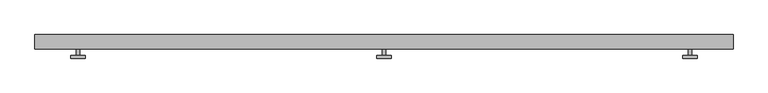
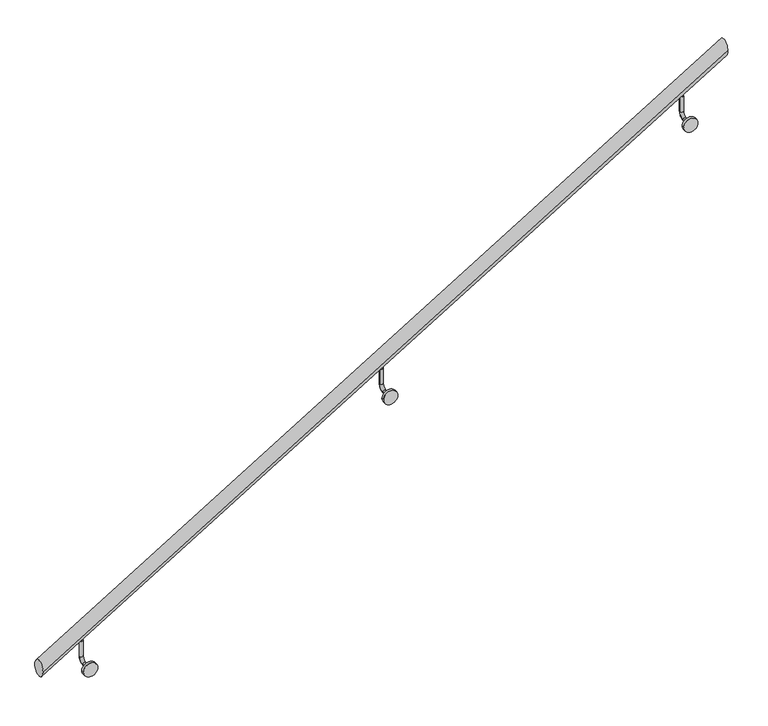
"""IFC4 building model written with IfcOpenShell, lengths in millimetres: railing geometry."""

from ifc_helpers import new_model, si_unit, point, frame, frame_2d, origin, place, context, project, spatial, circle_curve, ellipse_curve, trimmed, segment, composite_curve, outline, extrude, source, transform, mapped, element, save
from ifc_brep_helpers import plane_surface, cylinder_surface, revolved_surface, advanced_brep


def railing_4a983a7b(model_context):
    return source(origin(), model_context, "Body", "SolidModel", [
        advanced_brep(
        [(-49951.9507433, -7327.4994487, 6347.3929686), (-49951.9507433, -7377.4994487, 6347.3929686), (-47521.9507433, -7327.4994487, 7827.7377962), (-47521.9507433, -7377.4994487, 7827.7377962)],
        [
            (0, 1, ellipse_curve(frame((-49951.9507433, -7352.4994487, 6347.3929686), z_axis=(-1.0, 0.0, 0.0), x_axis=(0.0, 0.0, -1.0)), 29.2736981, 25.0)),
            (1, 0, ellipse_curve(frame((-49951.9507433, -7352.4994487, 6347.3929686), z_axis=(-1.0, 0.0, 0.0), x_axis=(0.0, 0.0, -1.0)), 29.2736981, 25.0)),
            (2, 3, ellipse_curve(frame((-47521.9507433, -7352.4994487, 7827.7377962), z_axis=(1.0, 0.0, 0.0), x_axis=(0.0, 0.0, -1.0)), 29.2736981, 25.0)),
            (3, 2, ellipse_curve(frame((-47521.9507433, -7352.4994487, 7827.7377962), z_axis=(1.0, 0.0, 0.0), x_axis=(0.0, 0.0, -1.0)), 29.2736981, 25.0)),
            (0, 2),
            (3, 1),
        ],
        [
            plane_surface(frame((-49951.9507433, -7352.4994487, 6376.6666667), z_axis=(-1.0, 0.0, 0.0), x_axis=(0.0, 1.0, 0.0))),
            plane_surface(frame((-47521.9507433, -7352.4994487, 7857.0114943), z_axis=(1.0, 0.0, 0.0), x_axis=(0.0, 1.0, 0.0))),
            cylinder_surface(frame((-49938.9442852, -7352.4994487, 6355.316443), z_axis=(-0.8540089447440427, 0.0, -0.5202583226601635), x_axis=(0.0, -1.0, 0.0)), 25.0),
        ],
        [
            (0, [[1, 2]]),
            (1, [[3, 4]]),
            (2, [[-1, 5, -4, 6]]),
            (2, [[-2, -6, -3, -5]]),
        ],
    ),
        advanced_brep(
        [(-48743.3007433, -7352.4994487, 7047.7890805), (-48730.6007433, -7352.4994487, 7047.7890805), (-48743.3007433, -7352.4994487, 6990.6390805), (-48730.6007433, -7352.4994487, 6990.6390805), (-48730.6007433, -7371.5494487, 6971.5890805), (-48743.3007433, -7371.5494487, 6971.5890805), (-48743.3007433, -7400.1244487, 6971.5890805), (-48730.6007433, -7400.1244487, 6971.5890805)],
        [
            (0, 1, circle_curve(frame((-48736.9507433, -7352.4994487, 7047.7890805), z_axis=(0.0, 0.0, 1.0), x_axis=(1.0, 0.0, 0.0)), 6.35)),
            (1, 0, circle_curve(frame((-48736.9507433, -7352.4994487, 7047.7890805), z_axis=(0.0, 0.0, 1.0), x_axis=(1.0, 0.0, 0.0)), 6.35)),
            (0, 2),
            (2, 3, circle_curve(frame((-48736.9507433, -7352.4994487, 6990.6390805), z_axis=(0.0, 0.0, 1.0), x_axis=(1.0, 0.0, 0.0)), 6.35)),
            (3, 1),
            (3, 2, circle_curve(frame((-48736.9507433, -7352.4994487, 6990.6390805), z_axis=(0.0, 0.0, 1.0), x_axis=(1.0, 0.0, 0.0)), 6.35)),
            (4, 3, circle_curve(frame((-48730.6007433, -7371.5494487, 6990.6390805), z_axis=(1.0, 0.0, 0.0), x_axis=(0.0, 1.0, 0.0)), 19.05)),
            (2, 5, circle_curve(frame((-48743.3007433, -7371.5494487, 6990.6390805), z_axis=(-1.0, 0.0, 0.0), x_axis=(0.0, 1.0, 0.0)), 19.05)),
            (5, 4, circle_curve(frame((-48736.9507433, -7371.5494487, 6971.5890805), z_axis=(0.0, 1.0, 0.0), x_axis=(1.0, 0.0, 0.0)), 6.35)),
            (4, 5, circle_curve(frame((-48736.9507433, -7371.5494487, 6971.5890805), z_axis=(0.0, 1.0, 0.0), x_axis=(1.0, 0.0, 0.0)), 6.35)),
            (6, 7, circle_curve(frame((-48736.9507433, -7400.1244487, 6971.5890805), z_axis=(0.0, -1.0, 0.0), x_axis=(1.0, 0.0, 0.0)), 6.35)),
            (7, 6, circle_curve(frame((-48736.9507433, -7400.1244487, 6971.5890805), z_axis=(0.0, -1.0, 0.0), x_axis=(1.0, 0.0, 0.0)), 6.35)),
            (5, 6),
            (7, 4),
        ],
        [
            plane_surface(frame((-48730.6007433, -7352.4994487, 7047.7890805), z_axis=(0.0, 0.0, 1.0), x_axis=(0.0, -1.0, 0.0))),
            cylinder_surface(frame((-48736.9507433, -7352.4994487, 7047.7890805), z_axis=(0.0, 0.0, 1.0), x_axis=(1.0, 0.0, 0.0)), 6.35),
            revolved_surface(trimmed(ellipse_curve(frame((-48736.9507433, -7352.4994487, 6990.6390805), z_axis=(0.0, 0.0, 1.0), x_axis=(1.0, 0.0, 0.0)), 6.35, 6.35), [point((-48743.3007433, -7352.4994487, 6990.6390805))], [point((-48730.6007433, -7352.4994487, 6990.6390805))], True, "CARTESIAN"), (-48736.9507433, -7371.5494487, 6990.6390805), (-1.0, 0.0, 0.0)),
            revolved_surface(trimmed(ellipse_curve(frame((-48736.9507433, -7352.4994487, 6990.6390805), z_axis=(0.0, 0.0, 1.0), x_axis=(1.0, 0.0, 0.0)), 6.35, 6.35), [point((-48730.6007433, -7352.4994487, 6990.6390805))], [point((-48743.3007433, -7352.4994487, 6990.6390805))], True, "CARTESIAN"), (-48736.9507433, -7371.5494487, 6990.6390805), (-1.0, 0.0, 0.0)),
            plane_surface(frame((-48736.9507433, -7400.1244487, 6965.2390805), z_axis=(0.0, -1.0, 0.0), x_axis=(1.0, 0.0, 0.0))),
            cylinder_surface(frame((-48736.9507433, -7371.5494487, 6971.5890805), z_axis=(0.0, 1.0, 0.0), x_axis=(1.0, 0.0, 0.0)), 6.35),
        ],
        [
            (0, [[1, 2]]),
            (1, [[-1, 3, 4, 5]]),
            (1, [[-2, -5, 6, -3]]),
            (2, [[7, -4, 8, 9]]),
            (3, [[-8, -6, -7, 10]]),
            (4, [[11, 12]]),
            (5, [[-9, 13, -12, 14]]),
            (5, [[-10, -14, -11, -13]]),
        ],
    ),
        extrude(outline(composite_curve([segment(trimmed(circle_curve(frame_2d((6971.5890805, -48736.9507433)), 25.4), [point((6971.5890805, -48711.5507433))], [point((6971.5890805, -48762.3507433))], False, "CARTESIAN"), True, "CONTINUOUS"), segment(trimmed(circle_curve(frame_2d((6971.5890805, -48736.9507433)), 25.4), [point((6971.5890805, -48762.3507433))], [point((6971.5890805, -48711.5507433))], False, "CARTESIAN"), True, "CONTINUOUS")], self_intersect=False)), frame((0.0, -7409.6494487, 0.0), z_axis=(0.0, 1.0, 0.0), x_axis=(0.0, 0.0, 1.0)), (0.0, 0.0, 1.0), 9.525),
        advanced_brep(
        [(-47678.3007433, -7352.4994487, 7696.5821839), (-47665.6007433, -7352.4994487, 7696.5821839), (-47678.3007433, -7352.4994487, 7639.4321839), (-47665.6007433, -7352.4994487, 7639.4321839), (-47665.6007433, -7371.5494487, 7620.3821839), (-47678.3007433, -7371.5494487, 7620.3821839), (-47678.3007433, -7400.1244487, 7620.3821839), (-47665.6007433, -7400.1244487, 7620.3821839)],
        [
            (0, 1, circle_curve(frame((-47671.9507433, -7352.4994487, 7696.5821839), z_axis=(0.0, 0.0, 1.0), x_axis=(1.0, 0.0, 0.0)), 6.35)),
            (1, 0, circle_curve(frame((-47671.9507433, -7352.4994487, 7696.5821839), z_axis=(0.0, 0.0, 1.0), x_axis=(1.0, 0.0, 0.0)), 6.35)),
            (0, 2),
            (2, 3, circle_curve(frame((-47671.9507433, -7352.4994487, 7639.4321839), z_axis=(0.0, 0.0, 1.0), x_axis=(1.0, 0.0, 0.0)), 6.35)),
            (3, 1),
            (3, 2, circle_curve(frame((-47671.9507433, -7352.4994487, 7639.4321839), z_axis=(0.0, 0.0, 1.0), x_axis=(1.0, 0.0, 0.0)), 6.35)),
            (4, 3, circle_curve(frame((-47665.6007433, -7371.5494487, 7639.4321839), z_axis=(1.0, 0.0, 0.0), x_axis=(0.0, 1.0, 0.0)), 19.05)),
            (2, 5, circle_curve(frame((-47678.3007433, -7371.5494487, 7639.4321839), z_axis=(-1.0, 0.0, 0.0), x_axis=(0.0, 1.0, 0.0)), 19.05)),
            (5, 4, circle_curve(frame((-47671.9507433, -7371.5494487, 7620.3821839), z_axis=(0.0, 1.0, 0.0), x_axis=(1.0, 0.0, 0.0)), 6.35)),
            (4, 5, circle_curve(frame((-47671.9507433, -7371.5494487, 7620.3821839), z_axis=(0.0, 1.0, 0.0), x_axis=(1.0, 0.0, 0.0)), 6.35)),
            (6, 7, circle_curve(frame((-47671.9507433, -7400.1244487, 7620.3821839), z_axis=(0.0, -1.0, 0.0), x_axis=(1.0, 0.0, 0.0)), 6.35)),
            (7, 6, circle_curve(frame((-47671.9507433, -7400.1244487, 7620.3821839), z_axis=(0.0, -1.0, 0.0), x_axis=(1.0, 0.0, 0.0)), 6.35)),
            (5, 6),
            (7, 4),
        ],
        [
            plane_surface(frame((-47665.6007433, -7352.4994487, 7696.5821839), z_axis=(0.0, 0.0, 1.0), x_axis=(0.0, -1.0, 0.0))),
            cylinder_surface(frame((-47671.9507433, -7352.4994487, 7696.5821839), z_axis=(0.0, 0.0, 1.0), x_axis=(1.0, 0.0, 0.0)), 6.35),
            revolved_surface(trimmed(ellipse_curve(frame((-47671.9507433, -7352.4994487, 7639.4321839), z_axis=(0.0, 0.0, 1.0), x_axis=(1.0, 0.0, 0.0)), 6.35, 6.35), [point((-47678.3007433, -7352.4994487, 7639.4321839))], [point((-47665.6007433, -7352.4994487, 7639.4321839))], True, "CARTESIAN"), (-47671.9507433, -7371.5494487, 7639.4321839), (-1.0, 0.0, 0.0)),
            revolved_surface(trimmed(ellipse_curve(frame((-47671.9507433, -7352.4994487, 7639.4321839), z_axis=(0.0, 0.0, 1.0), x_axis=(1.0, 0.0, 0.0)), 6.35, 6.35), [point((-47665.6007433, -7352.4994487, 7639.4321839))], [point((-47678.3007433, -7352.4994487, 7639.4321839))], True, "CARTESIAN"), (-47671.9507433, -7371.5494487, 7639.4321839), (-1.0, 0.0, 0.0)),
            plane_surface(frame((-47671.9507433, -7400.1244487, 7614.0321839), z_axis=(0.0, -1.0, 0.0), x_axis=(1.0, 0.0, 0.0))),
            cylinder_surface(frame((-47671.9507433, -7371.5494487, 7620.3821839), z_axis=(0.0, 1.0, 0.0), x_axis=(1.0, 0.0, 0.0)), 6.35),
        ],
        [
            (0, [[1, 2]]),
            (1, [[-1, 3, 4, 5]]),
            (1, [[-2, -5, 6, -3]]),
            (2, [[7, -4, 8, 9]]),
            (3, [[-8, -6, -7, 10]]),
            (4, [[11, 12]]),
            (5, [[-9, 13, -12, 14]]),
            (5, [[-10, -14, -11, -13]]),
        ],
    ),
        extrude(outline(composite_curve([segment(trimmed(circle_curve(frame_2d((7620.3821839, -47671.9507433)), 25.4), [point((7620.3821839, -47646.5507433))], [point((7620.3821839, -47697.3507433))], False, "CARTESIAN"), True, "CONTINUOUS"), segment(trimmed(circle_curve(frame_2d((7620.3821839, -47671.9507433)), 25.4), [point((7620.3821839, -47697.3507433))], [point((7620.3821839, -47646.5507433))], False, "CARTESIAN"), True, "CONTINUOUS")], self_intersect=False)), frame((0.0, -7409.6494487, 0.0), z_axis=(0.0, 1.0, 0.0), x_axis=(0.0, 0.0, 1.0)), (0.0, 0.0, 1.0), 9.525),
        advanced_brep(
        [(-49808.3007433, -7352.4994487, 6398.995977), (-49795.6007433, -7352.4994487, 6398.995977), (-49808.3007433, -7352.4994487, 6341.845977), (-49795.6007433, -7352.4994487, 6341.845977), (-49795.6007433, -7371.5494487, 6322.795977), (-49808.3007433, -7371.5494487, 6322.795977), (-49808.3007433, -7400.1244487, 6322.795977), (-49795.6007433, -7400.1244487, 6322.795977)],
        [
            (0, 1, circle_curve(frame((-49801.9507433, -7352.4994487, 6398.995977), z_axis=(0.0, 0.0, 1.0), x_axis=(1.0, 0.0, 0.0)), 6.35)),
            (1, 0, circle_curve(frame((-49801.9507433, -7352.4994487, 6398.995977), z_axis=(0.0, 0.0, 1.0), x_axis=(1.0, 0.0, 0.0)), 6.35)),
            (0, 2),
            (2, 3, circle_curve(frame((-49801.9507433, -7352.4994487, 6341.845977), z_axis=(0.0, 0.0, 1.0), x_axis=(1.0, 0.0, 0.0)), 6.35)),
            (3, 1),
            (3, 2, circle_curve(frame((-49801.9507433, -7352.4994487, 6341.845977), z_axis=(0.0, 0.0, 1.0), x_axis=(1.0, 0.0, 0.0)), 6.35)),
            (4, 3, circle_curve(frame((-49795.6007433, -7371.5494487, 6341.845977), z_axis=(1.0, 0.0, 0.0), x_axis=(0.0, 1.0, 0.0)), 19.05)),
            (2, 5, circle_curve(frame((-49808.3007433, -7371.5494487, 6341.845977), z_axis=(-1.0, 0.0, 0.0), x_axis=(0.0, 1.0, 0.0)), 19.05)),
            (5, 4, circle_curve(frame((-49801.9507433, -7371.5494487, 6322.795977), z_axis=(0.0, 1.0, 0.0), x_axis=(1.0, 0.0, 0.0)), 6.35)),
            (4, 5, circle_curve(frame((-49801.9507433, -7371.5494487, 6322.795977), z_axis=(0.0, 1.0, 0.0), x_axis=(1.0, 0.0, 0.0)), 6.35)),
            (6, 7, circle_curve(frame((-49801.9507433, -7400.1244487, 6322.795977), z_axis=(0.0, -1.0, 0.0), x_axis=(1.0, 0.0, 0.0)), 6.35)),
            (7, 6, circle_curve(frame((-49801.9507433, -7400.1244487, 6322.795977), z_axis=(0.0, -1.0, 0.0), x_axis=(1.0, 0.0, 0.0)), 6.35)),
            (5, 6),
            (7, 4),
        ],
        [
            plane_surface(frame((-49795.6007433, -7352.4994487, 6398.995977), z_axis=(0.0, 0.0, 1.0), x_axis=(0.0, -1.0, 0.0))),
            cylinder_surface(frame((-49801.9507433, -7352.4994487, 6398.995977), z_axis=(0.0, 0.0, 1.0), x_axis=(1.0, 0.0, 0.0)), 6.35),
            revolved_surface(trimmed(ellipse_curve(frame((-49801.9507433, -7352.4994487, 6341.845977), z_axis=(0.0, 0.0, 1.0), x_axis=(1.0, 0.0, 0.0)), 6.35, 6.35), [point((-49808.3007433, -7352.4994487, 6341.845977))], [point((-49795.6007433, -7352.4994487, 6341.845977))], True, "CARTESIAN"), (-49801.9507433, -7371.5494487, 6341.845977), (-1.0, 0.0, 0.0)),
            revolved_surface(trimmed(ellipse_curve(frame((-49801.9507433, -7352.4994487, 6341.845977), z_axis=(0.0, 0.0, 1.0), x_axis=(1.0, 0.0, 0.0)), 6.35, 6.35), [point((-49795.6007433, -7352.4994487, 6341.845977))], [point((-49808.3007433, -7352.4994487, 6341.845977))], True, "CARTESIAN"), (-49801.9507433, -7371.5494487, 6341.845977), (-1.0, 0.0, 0.0)),
            plane_surface(frame((-49801.9507433, -7400.1244487, 6316.445977), z_axis=(0.0, -1.0, 0.0), x_axis=(1.0, 0.0, 0.0))),
            cylinder_surface(frame((-49801.9507433, -7371.5494487, 6322.795977), z_axis=(0.0, 1.0, 0.0), x_axis=(1.0, 0.0, 0.0)), 6.35),
        ],
        [
            (0, [[1, 2]]),
            (1, [[-1, 3, 4, 5]]),
            (1, [[-2, -5, 6, -3]]),
            (2, [[7, -4, 8, 9]]),
            (3, [[-8, -6, -7, 10]]),
            (4, [[11, 12]]),
            (5, [[-9, 13, -12, 14]]),
            (5, [[-10, -14, -11, -13]]),
        ],
    ),
        extrude(outline(composite_curve([segment(trimmed(circle_curve(frame_2d((6322.795977, -49801.9507433)), 25.4), [point((6322.795977, -49776.5507433))], [point((6322.795977, -49827.3507433))], False, "CARTESIAN"), True, "CONTINUOUS"), segment(trimmed(circle_curve(frame_2d((6322.795977, -49801.9507433)), 25.4), [point((6322.795977, -49827.3507433))], [point((6322.795977, -49776.5507433))], False, "CARTESIAN"), True, "CONTINUOUS")], self_intersect=False)), frame((0.0, -7409.6494487, 0.0), z_axis=(0.0, 1.0, 0.0), x_axis=(0.0, 0.0, 1.0)), (0.0, 0.0, 1.0), 9.525),
    ])


if __name__ == "__main__":
    model = new_model("IFC4")
    model_context = context("Model", 3, world=origin())
    ifc_project = project(units=[si_unit("LENGTHUNIT", "METRE", prefix="MILLI")], contexts=[model_context])
    site = spatial("IfcSite", under=ifc_project)
    building = spatial("IfcBuilding", under=site)
    placement = place(None, origin())
    railing_shape = railing_4a983a7b(model_context)
    element("IfcRailing", 1, at=placement, inside=building, context=model_context, shape_type="MappedRepresentation", body=[
        mapped(railing_shape, transform((0.0, 0.0, 0.0), x_axis=(1.0, 0.0, 0.0), y_axis=(0.0, 1.0, 0.0), z_axis=(0.0, 0.0, 1.0))),
    ])
    save(model, "model.ifc")
